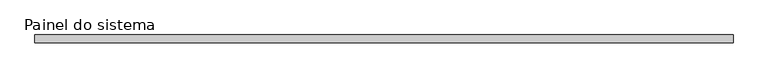
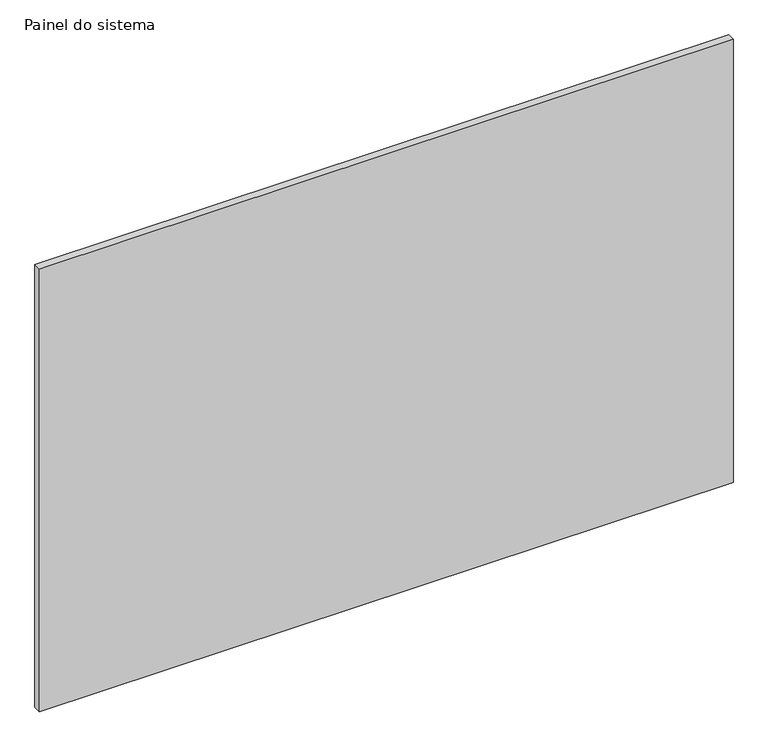
"""IFC4 building model written with IfcOpenShell, lengths in millimetres: plate geometry, Painel do sistema : Envidraçado."""

from ifc_helpers import new_model, si_unit, origin, origin_with_axes, place, context, project, spatial, polyline, outline, extrude, source, transform, mapped, element, save


def painel_do_sistema_91df381f(model_context):
    return source(origin(), model_context, "Body", "SweptSolid", [
        extrude(outline(polyline([(1110.3819696, -49.5), (-1110.3819696, -49.5), (-1110.3819696, -24.5), (1110.3819696, -24.5), (1110.3819696, -49.5)])), origin_with_axes(), (0.0, 0.0, 1.0), 1500.0),
    ])


if __name__ == "__main__":
    model = new_model("IFC4")
    model_context = context("Model", 3, world=origin())
    ifc_project = project(units=[si_unit("LENGTHUNIT", "METRE", prefix="MILLI")], contexts=[model_context])
    site = spatial("IfcSite", under=ifc_project)
    building = spatial("IfcBuilding", under=site)
    placement = place(None, origin())
    painel_do_sistema_shape = painel_do_sistema_91df381f(model_context)
    element("IfcPlate", 1, ObjectType="Painel do sistema : Envidraçado", at=placement, inside=building, context=model_context, shape_type="MappedRepresentation", body=[
        mapped(painel_do_sistema_shape, transform((0.0, 0.0, 0.0), x_axis=(1.0, 0.0, 0.0), y_axis=(0.0, 1.0, 0.0), z_axis=(0.0, 0.0, 1.0))),
    ])
    save(model, "model.ifc")

# Revit data of these elements
# Type "Painel do sistema : Envidraçado"
#   Construction Type Id = "GSP4R"
#   Analytic Construction = "Vidraça única Pilkington 1/8 pol"
#   Visual Light Transmittance = 0.9
#   Solar Heat Gain Coefficient = 0.86
#   Heat Transfer Coefficient (U) = 6.7069 W/(m²·K)
# Element 1 (IfcPlate, "Painel do sistema : Envidraçado")
#   Materials on its faces: "Vidro"
# Materials
#   "Vidro": class "Vidro", colour RGB 0 128 192, transparency 0.9, Description = "Vidro de sílica", Cost = 0
